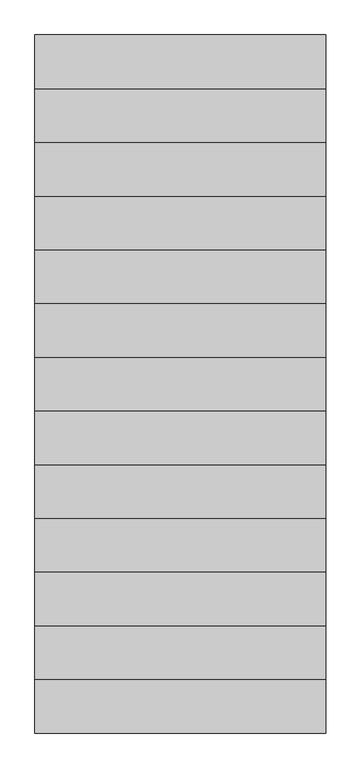
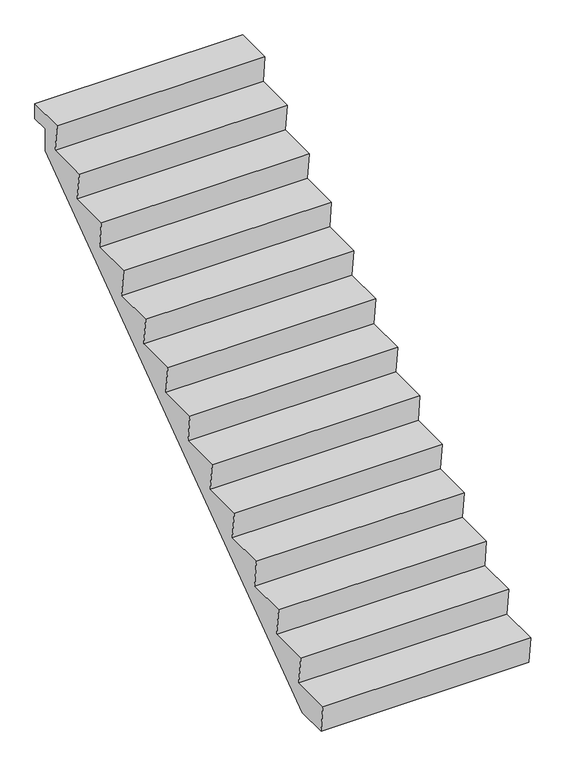
"""IFC4 building model written with IfcOpenShell, lengths in millimetres: proxy geometry, NLRS_24_GM_LB_rechte steektrap prefab-AV_gen_rsf : prefab trap_gen__aant=12 b=1200 a=220 o=172.7 zonder bomen."""

from ifc_helpers import new_model, si_unit, frame, origin, place, context, project, spatial, polyline, outline, extrude, source, transform, mapped, element, save


def generic_models_322cbe82(model_context):
    return source(origin(), model_context, "Body", "SweptSolid", [
        extrude(outline(polyline([(2880.0, 2270.0), (3120.0, 2270.0), (3120.0, 2170.0), (3010.0, 2170.0), (3010.0, 2027.0164203), (223.9686206, 0.0), (20.0, 0.0), (0.0, 174.6153846), (260.0, 174.6153846), (240.0, 349.2307692), (500.0, 349.2307692), (480.0, 523.8461538), (740.0, 523.8461538), (720.0, 698.4615385), (980.0, 698.4615385), (960.0, 873.0769231), (1220.0, 873.0769231), (1200.0, 1047.6923077), (1460.0, 1047.6923077), (1440.0, 1222.3076923), (1700.0, 1222.3076923), (1680.0, 1396.9230769), (1940.0, 1396.9230769), (1920.0, 1571.5384615), (2180.0, 1571.5384615), (2160.0, 1746.1538462), (2420.0, 1746.1538462), (2400.0, 1920.7692308), (2660.0, 1920.7692308), (2640.0, 2095.3846154), (2900.0, 2095.3846154), (2880.0, 2270.0)])), frame((-650.0, 0.0, 0.0), z_axis=(1.0, 0.0, 0.0), x_axis=(0.0, 1.0, 0.0)), (0.0, 0.0, 1.0), 1300.0),
    ])


if __name__ == "__main__":
    model = new_model("IFC4")
    model_context = context("Model", 3, world=origin())
    ifc_project = project(units=[si_unit("LENGTHUNIT", "METRE", prefix="MILLI")], contexts=[model_context])
    site = spatial("IfcSite", under=ifc_project)
    building = spatial("IfcBuilding", under=site)
    placement = place(None, origin())
    generic_models_shape = generic_models_322cbe82(model_context)
    element("IfcBuildingElementProxy", 1, Name="NLRS_24_GM_LB_rechte steektrap prefab-AV_gen_rsf : prefab trap_gen__aant=12 b=1200 a=220 o=172.7 zonder bomen", ObjectType="NLRS_24_GM_LB_rechte steektrap prefab-AV_gen_rsf : prefab trap_gen__aant=12 b=1200 a=220 o=172.7 zonder bomen", at=placement, inside=building, context=model_context, shape_type="MappedRepresentation", body=[
        mapped(generic_models_shape, transform((0.0, 0.0, 0.0), x_axis=(1.0, 0.0, 0.0), y_axis=(0.0, 1.0, 0.0), z_axis=(0.0, 0.0, 1.0))),
    ])
    save(model, "model.ifc")

# Revit data of these elements
# Type "NLRS_24_GM_LB_rechte steektrap prefab-AV_gen_rsf : prefab trap_gen__aant=12 b=1200 a=220 o=172.7 zonder bomen"
#   Export Type to IFC As = "IfcStair"
#   Type IfcGUID = "2CEqVLPNH8KRN7ghwV3ZFx"
#   Type Comments = " "
#   Model = " "
#   Manufacturer = " "
#   Keynote = " "
#   Description = "rechte steektrap prefab\r\naant=11 b=1200 a=220 o=181,8\r\nzonder bomen"
#   Assembly Code = "24.11"
#   Aantrede onder = 240 mm
#   Width = 1300 mm
#   Wel diepte = 20 mm
#   Trapboom breedte = 0 mm
#   Thickness = 120 mm
#   Optrede onderste trede = 150 mm
#   NLRS_C_lengte = 2880 mm
#   Length = 3360 mm
#   Hoogte oplegnok onder = 100 mm
#   Hoogte oplegnok boven = 100 mm
#   Height = 2270 mm
#   Breedte oplegnok boven = 110 mm
#   BottomCalc = 150 mm
#   Actual Tread Depth = 240 mm
#   Actual Riser Height = 174.615 mm
#   Actual Number of Tread = 12
#   Actual Number of Risers = 13
#   Aantrede boven = 240 mm
#   Aantal treden max dertig = 13
#   Trapboom = no
#   Oplegnok onder = no
#   NLRS_C_materiaal = NLRS_f2_beton prefab_gen_rsf
#   Default Elevation = 0
# Element 1 (IfcBuildingElementProxy, "NLRS_24_GM_LB_rechte steektrap prefab-AV_gen_rsf : prefab trap_gen__aant=12 b=1200 a=220 o=172.7 zonder bomen")
#   Materials on its faces: "NLRS_f2_beton prefab_gen_rsf"
# Materials
#   "NLRS_f2_beton prefab_gen_rsf": class "F - Niet gebakken kunststeen", colour RGB 129 133 118, transparency 0, Keynote = "f2", Manufacturer = "Revit Standards Foundation", URL = "www.revitstandards.org", Description = "beton prefab", Cost = 0
